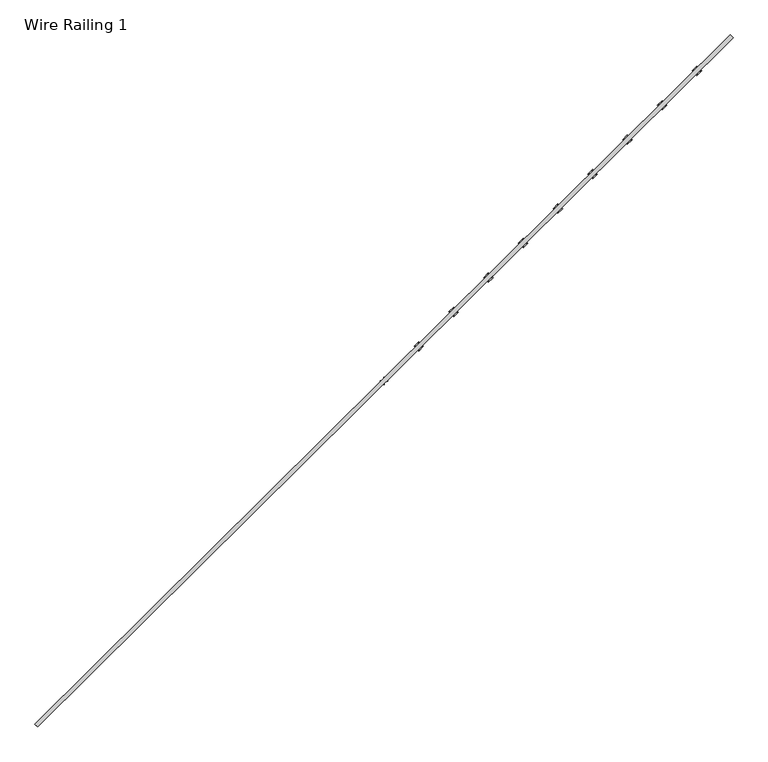
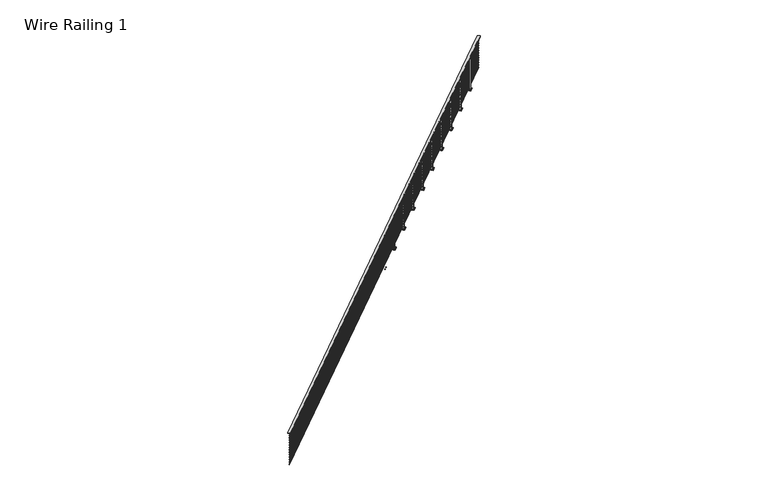
"""IFC4 building model written with IfcOpenShell, lengths in millimetres: railing geometry, Wire Railing 1."""

from ifc_helpers import new_model, si_unit, point, frame, frame_2d, origin, place, context, project, spatial, polyline, circle_curve, trimmed, segment, composite_curve, outline, extrude, source, transform, mapped, element, save


def wire_railing_1_bdb17c3e(model_context):
    return source(origin(), model_context, "Body", "SweptSolid", [
        extrude(outline(polyline([(32583.8298074, 24310.825617), (32530.1909697, 24364.9487644), (45743.1001377, 37459.6249857), (45796.7389755, 37405.5018383), (32583.8298074, 24310.825617)])), frame((0.0, 0.0, 265004.55), z_axis=(0.0, 0.0, 1.0), x_axis=(1.0, 0.0, 0.0)), (0.0, 0.0, 1.0), 19.05),
        extrude(outline(composite_curve([segment(trimmed(circle_curve(frame_2d((0.0, 2.38125)), 2.38125), [point((-2.38125, 2.38125))], [point((2.38125, 2.38125))], False, "CARTESIAN"), True, "CONTINUOUS"), segment(trimmed(circle_curve(frame_2d((0.0, 2.38125)), 2.38125), [point((2.38125, 2.38125))], [point((-2.38125, 2.38125))], False, "CARTESIAN"), True, "CONTINUOUS")], self_intersect=False)), frame((32557.0103886, 24337.8871907, 264947.4), z_axis=(0.7102775248505508, 0.7039217553763878, 0.0), x_axis=(0.7039217553763878, -0.7102775248505508, 0.0)), (0.0, 0.0, 1.0), 18602.4598918),
        extrude(outline(composite_curve([segment(trimmed(circle_curve(frame_2d((0.0, 2.38125)), 2.38125), [point((-2.38125, 2.38125))], [point((2.38125, 2.38125))], False, "CARTESIAN"), True, "CONTINUOUS"), segment(trimmed(circle_curve(frame_2d((0.0, 2.38125)), 2.38125), [point((2.38125, 2.38125))], [point((-2.38125, 2.38125))], False, "CARTESIAN"), True, "CONTINUOUS")], self_intersect=False)), frame((32557.0103886, 24337.8871907, 264871.2), z_axis=(0.7102775248505508, 0.7039217553763878, 0.0), x_axis=(0.7039217553763878, -0.7102775248505508, 0.0)), (0.0, 0.0, 1.0), 18602.4598918),
        extrude(outline(composite_curve([segment(trimmed(circle_curve(frame_2d((0.0, 2.38125)), 2.38125), [point((-2.38125, 2.38125))], [point((2.38125, 2.38125))], False, "CARTESIAN"), True, "CONTINUOUS"), segment(trimmed(circle_curve(frame_2d((0.0, 2.38125)), 2.38125), [point((2.38125, 2.38125))], [point((-2.38125, 2.38125))], False, "CARTESIAN"), True, "CONTINUOUS")], self_intersect=False)), frame((32557.0103886, 24337.8871907, 264795.0), z_axis=(0.7102775248505508, 0.7039217553763878, 0.0), x_axis=(0.7039217553763878, -0.7102775248505508, 0.0)), (0.0, 0.0, 1.0), 18602.4598918),
        extrude(outline(composite_curve([segment(trimmed(circle_curve(frame_2d((0.0, 2.38125)), 2.38125), [point((-2.38125, 2.38125))], [point((2.38125, 2.38125))], False, "CARTESIAN"), True, "CONTINUOUS"), segment(trimmed(circle_curve(frame_2d((0.0, 2.38125)), 2.38125), [point((2.38125, 2.38125))], [point((-2.38125, 2.38125))], False, "CARTESIAN"), True, "CONTINUOUS")], self_intersect=False)), frame((32557.0103886, 24337.8871907, 264718.8), z_axis=(0.7102775248505508, 0.7039217553763878, 0.0), x_axis=(0.7039217553763878, -0.7102775248505508, 0.0)), (0.0, 0.0, 1.0), 18602.4598918),
        extrude(outline(composite_curve([segment(trimmed(circle_curve(frame_2d((0.0, 2.38125)), 2.38125), [point((-2.38125, 2.38125))], [point((2.38125, 2.38125))], False, "CARTESIAN"), True, "CONTINUOUS"), segment(trimmed(circle_curve(frame_2d((0.0, 2.38125)), 2.38125), [point((2.38125, 2.38125))], [point((-2.38125, 2.38125))], False, "CARTESIAN"), True, "CONTINUOUS")], self_intersect=False)), frame((32557.0103886, 24337.8871907, 264642.6), z_axis=(0.7102775248505508, 0.7039217553763878, 0.0), x_axis=(0.7039217553763878, -0.7102775248505508, 0.0)), (0.0, 0.0, 1.0), 18602.4598918),
        extrude(outline(composite_curve([segment(trimmed(circle_curve(frame_2d((0.0, 2.38125)), 2.38125), [point((-2.38125, 2.38125))], [point((2.38125, 2.38125))], False, "CARTESIAN"), True, "CONTINUOUS"), segment(trimmed(circle_curve(frame_2d((0.0, 2.38125)), 2.38125), [point((2.38125, 2.38125))], [point((-2.38125, 2.38125))], False, "CARTESIAN"), True, "CONTINUOUS")], self_intersect=False)), frame((32557.0103886, 24337.8871907, 264566.4), z_axis=(0.7102775248505508, 0.7039217553763878, 0.0), x_axis=(0.7039217553763878, -0.7102775248505508, 0.0)), (0.0, 0.0, 1.0), 18602.4598918),
        extrude(outline(composite_curve([segment(trimmed(circle_curve(frame_2d((0.0, 2.38125)), 2.38125), [point((-2.38125, 2.38125))], [point((2.38125, 2.38125))], False, "CARTESIAN"), True, "CONTINUOUS"), segment(trimmed(circle_curve(frame_2d((0.0, 2.38125)), 2.38125), [point((2.38125, 2.38125))], [point((-2.38125, 2.38125))], False, "CARTESIAN"), True, "CONTINUOUS")], self_intersect=False)), frame((32557.0103886, 24337.8871907, 264490.2), z_axis=(0.7102775248505508, 0.7039217553763878, 0.0), x_axis=(0.7039217553763878, -0.7102775248505508, 0.0)), (0.0, 0.0, 1.0), 18602.4598918),
        extrude(outline(composite_curve([segment(trimmed(circle_curve(frame_2d((0.0, 2.38125)), 2.38125), [point((-2.38125, 2.38125))], [point((2.38125, 2.38125))], False, "CARTESIAN"), True, "CONTINUOUS"), segment(trimmed(circle_curve(frame_2d((0.0, 2.38125)), 2.38125), [point((2.38125, 2.38125))], [point((-2.38125, 2.38125))], False, "CARTESIAN"), True, "CONTINUOUS")], self_intersect=False)), frame((32557.0103886, 24337.8871907, 264414.0), z_axis=(0.7102775248505508, 0.7039217553763878, 0.0), x_axis=(0.7039217553763878, -0.7102775248505508, 0.0)), (0.0, 0.0, 1.0), 18602.4598918),
        extrude(outline(composite_curve([segment(trimmed(circle_curve(frame_2d((0.0, 2.38125)), 2.38125), [point((-2.38125, 2.38125))], [point((2.38125, 2.38125))], False, "CARTESIAN"), True, "CONTINUOUS"), segment(trimmed(circle_curve(frame_2d((0.0, 2.38125)), 2.38125), [point((2.38125, 2.38125))], [point((-2.38125, 2.38125))], False, "CARTESIAN"), True, "CONTINUOUS")], self_intersect=False)), frame((32557.0103886, 24337.8871907, 264337.8), z_axis=(0.7102775248505508, 0.7039217553763878, 0.0), x_axis=(0.7039217553763878, -0.7102775248505508, 0.0)), (0.0, 0.0, 1.0), 18602.4598918),
        extrude(outline(composite_curve([segment(trimmed(circle_curve(frame_2d((0.0, 2.38125)), 2.38125), [point((-2.38125, 2.38125))], [point((2.38125, 2.38125))], False, "CARTESIAN"), True, "CONTINUOUS"), segment(trimmed(circle_curve(frame_2d((0.0, 2.38125)), 2.38125), [point((2.38125, 2.38125))], [point((-2.38125, 2.38125))], False, "CARTESIAN"), True, "CONTINUOUS")], self_intersect=False)), frame((32557.0103886, 24337.8871907, 264261.6), z_axis=(0.7102775248505508, 0.7039217553763878, 0.0), x_axis=(0.7039217553763878, -0.7102775248505508, 0.0)), (0.0, 0.0, 1.0), 18602.4598918),
        extrude(outline(composite_curve([segment(trimmed(circle_curve(frame_2d((0.0, 2.38125)), 2.38125), [point((-2.38125, 2.38125))], [point((2.38125, 2.38125))], False, "CARTESIAN"), True, "CONTINUOUS"), segment(trimmed(circle_curve(frame_2d((0.0, 2.38125)), 2.38125), [point((2.38125, 2.38125))], [point((-2.38125, 2.38125))], False, "CARTESIAN"), True, "CONTINUOUS")], self_intersect=False)), frame((32557.0103886, 24337.8871907, 264185.4), z_axis=(0.7102775248505508, 0.7039217553763878, 0.0), x_axis=(0.7039217553763878, -0.7102775248505508, 0.0)), (0.0, 0.0, 1.0), 18602.4598918),
        extrude(outline(composite_curve([segment(trimmed(circle_curve(frame_2d((0.0, 2.38125)), 2.38125), [point((-2.38125, 2.38125))], [point((2.38125, 2.38125))], False, "CARTESIAN"), True, "CONTINUOUS"), segment(trimmed(circle_curve(frame_2d((0.0, 2.38125)), 2.38125), [point((2.38125, 2.38125))], [point((-2.38125, 2.38125))], False, "CARTESIAN"), True, "CONTINUOUS")], self_intersect=False)), frame((32557.0103886, 24337.8871907, 264109.2), z_axis=(0.7102775248505508, 0.7039217553763878, 0.0), x_axis=(0.7039217553763878, -0.7102775248505508, 0.0)), (0.0, 0.0, 1.0), 18602.4598918),
        extrude(outline(composite_curve([segment(trimmed(circle_curve(frame_2d((0.0, 2.38125)), 2.38125), [point((-2.38125, 2.38125))], [point((2.38125, 2.38125))], False, "CARTESIAN"), True, "CONTINUOUS"), segment(trimmed(circle_curve(frame_2d((0.0, 2.38125)), 2.38125), [point((2.38125, 2.38125))], [point((-2.38125, 2.38125))], False, "CARTESIAN"), True, "CONTINUOUS")], self_intersect=False)), frame((32557.0103886, 24337.8871907, 264033.0), z_axis=(0.7102775248505508, 0.7039217553763878, 0.0), x_axis=(0.7039217553763878, -0.7102775248505508, 0.0)), (0.0, 0.0, 1.0), 18602.4598918),
        extrude(outline(composite_curve([segment(trimmed(circle_curve(frame_2d((45108.9915842, 36714.968443)), 6.35), [point((45113.4614874, 36710.4581807))], [point((45104.5216811, 36719.4787052))], False, "CARTESIAN"), True, "CONTINUOUS"), segment(trimmed(circle_curve(frame_2d((45108.9915842, 36714.968443)), 6.35), [point((45104.5216811, 36719.4787052))], [point((45113.4614874, 36710.4581807))], False, "CARTESIAN"), True, "CONTINUOUS")], self_intersect=False)), frame((0.0, 0.0, 263956.8), z_axis=(0.0, 0.0, 1.0), x_axis=(1.0, 0.0, 0.0)), (0.0, 0.0, 1.0), 12.7),
        extrude(outline(composite_curve([segment(trimmed(circle_curve(frame_2d((45046.4129402, 36778.1121149)), 6.35), [point((45050.8828433, 36773.6018526))], [point((45041.943037, 36782.6223772))], False, "CARTESIAN"), True, "CONTINUOUS"), segment(trimmed(circle_curve(frame_2d((45046.4129402, 36778.1121149)), 6.35), [point((45041.943037, 36782.6223772))], [point((45050.8828433, 36773.6018526))], False, "CARTESIAN"), True, "CONTINUOUS")], self_intersect=False)), frame((0.0, 0.0, 263956.8), z_axis=(0.0, 0.0, 1.0), x_axis=(1.0, 0.0, 0.0)), (0.0, 0.0, 1.0), 12.7),
        extrude(outline(composite_curve([segment(trimmed(circle_curve(frame_2d((45172.1352562, 36777.547087)), 6.35), [point((45176.6051594, 36773.0368247))], [point((45167.6653531, 36782.0573493))], False, "CARTESIAN"), True, "CONTINUOUS"), segment(trimmed(circle_curve(frame_2d((45172.1352562, 36777.547087)), 6.35), [point((45167.6653531, 36782.0573493))], [point((45176.6051594, 36773.0368247))], False, "CARTESIAN"), True, "CONTINUOUS")], self_intersect=False)), frame((0.0, 0.0, 263956.8), z_axis=(0.0, 0.0, 1.0), x_axis=(1.0, 0.0, 0.0)), (0.0, 0.0, 1.0), 12.7),
        extrude(outline(composite_curve([segment(trimmed(circle_curve(frame_2d((45109.5566122, 36840.690759)), 6.35), [point((45114.0265153, 36836.1804967))], [point((45105.086709, 36845.2010212))], False, "CARTESIAN"), True, "CONTINUOUS"), segment(trimmed(circle_curve(frame_2d((45109.5566122, 36840.690759)), 6.35), [point((45105.086709, 36845.2010212))], [point((45114.0265153, 36836.1804967))], False, "CARTESIAN"), True, "CONTINUOUS")], self_intersect=False)), frame((0.0, 0.0, 263956.8), z_axis=(0.0, 0.0, 1.0), x_axis=(1.0, 0.0, 0.0)), (0.0, 0.0, 1.0), 12.7),
        extrude(outline(polyline([(45019.4724439, 36778.2331923), (45109.6776896, 36867.6312553), (45199.0757525, 36777.4260096), (45108.8705068, 36688.0279467), (45019.4724439, 36778.2331923)])), frame((0.0, 0.0, 263956.8), z_axis=(0.0, 0.0, 1.0), x_axis=(1.0, 0.0, 0.0)), (0.0, 0.0, 1.0), 6.35),
        extrude(outline(polyline([(45066.6183124, 36778.0213069), (45109.4658041, 36820.4853867), (45151.929884, 36777.6378951), (45109.0823923, 36735.1738152), (45066.6183124, 36778.0213069)]), holes=[polyline([(45075.5984778, 36777.9809477), (45109.1227514, 36744.1539806), (45142.9497186, 36777.6782542), (45109.425445, 36811.5052213), (45075.5984778, 36777.9809477)])]), frame((0.0, 0.0, 263956.8), z_axis=(0.0, 0.0, 1.0), x_axis=(1.0, 0.0, 0.0)), (0.0, 0.0, 1.0), 1047.75),
        extrude(outline(composite_curve([segment(trimmed(circle_curve(frame_2d((44448.3461258, 36060.2346319)), 6.35), [point((44452.816029, 36055.7243696))], [point((44443.8762227, 36064.7448942))], False, "CARTESIAN"), True, "CONTINUOUS"), segment(trimmed(circle_curve(frame_2d((44448.3461258, 36060.2346319)), 6.35), [point((44443.8762227, 36064.7448942))], [point((44452.816029, 36055.7243696))], False, "CARTESIAN"), True, "CONTINUOUS")], self_intersect=False)), frame((0.0, 0.0, 263956.8), z_axis=(0.0, 0.0, 1.0), x_axis=(1.0, 0.0, 0.0)), (0.0, 0.0, 1.0), 12.7),
        extrude(outline(composite_curve([segment(trimmed(circle_curve(frame_2d((44385.7674818, 36123.3783038)), 6.35), [point((44390.2373849, 36118.8680416))], [point((44381.2975786, 36127.8885661))], False, "CARTESIAN"), True, "CONTINUOUS"), segment(trimmed(circle_curve(frame_2d((44385.7674818, 36123.3783038)), 6.35), [point((44381.2975786, 36127.8885661))], [point((44390.2373849, 36118.8680416))], False, "CARTESIAN"), True, "CONTINUOUS")], self_intersect=False)), frame((0.0, 0.0, 263956.8), z_axis=(0.0, 0.0, 1.0), x_axis=(1.0, 0.0, 0.0)), (0.0, 0.0, 1.0), 12.7),
        extrude(outline(composite_curve([segment(trimmed(circle_curve(frame_2d((44511.4897978, 36122.8132759)), 6.35), [point((44515.959701, 36118.3030137))], [point((44507.0198947, 36127.3235382))], False, "CARTESIAN"), True, "CONTINUOUS"), segment(trimmed(circle_curve(frame_2d((44511.4897978, 36122.8132759)), 6.35), [point((44507.0198947, 36127.3235382))], [point((44515.959701, 36118.3030137))], False, "CARTESIAN"), True, "CONTINUOUS")], self_intersect=False)), frame((0.0, 0.0, 263956.8), z_axis=(0.0, 0.0, 1.0), x_axis=(1.0, 0.0, 0.0)), (0.0, 0.0, 1.0), 12.7),
        extrude(outline(composite_curve([segment(trimmed(circle_curve(frame_2d((44448.9111538, 36185.9569479)), 6.35), [point((44453.3810569, 36181.4466856))], [point((44444.4412506, 36190.4672102))], False, "CARTESIAN"), True, "CONTINUOUS"), segment(trimmed(circle_curve(frame_2d((44448.9111538, 36185.9569479)), 6.35), [point((44444.4412506, 36190.4672102))], [point((44453.3810569, 36181.4466856))], False, "CARTESIAN"), True, "CONTINUOUS")], self_intersect=False)), frame((0.0, 0.0, 263956.8), z_axis=(0.0, 0.0, 1.0), x_axis=(1.0, 0.0, 0.0)), (0.0, 0.0, 1.0), 12.7),
        extrude(outline(polyline([(44358.8269855, 36123.4993813), (44449.0322312, 36212.8974442), (44538.4302941, 36122.6921985), (44448.2250484, 36033.2941356), (44358.8269855, 36123.4993813)])), frame((0.0, 0.0, 263956.8), z_axis=(0.0, 0.0, 1.0), x_axis=(1.0, 0.0, 0.0)), (0.0, 0.0, 1.0), 6.35),
        extrude(outline(polyline([(44405.972854, 36123.2874958), (44448.8203457, 36165.7515757), (44491.2844256, 36122.904084), (44448.4369339, 36080.4400041), (44405.972854, 36123.2874958)]), holes=[polyline([(44414.9530194, 36123.2471367), (44448.477293, 36089.4201695), (44482.3042602, 36122.9444431), (44448.7799866, 36156.7714103), (44414.9530194, 36123.2471367)])]), frame((0.0, 0.0, 263956.8), z_axis=(0.0, 0.0, 1.0), x_axis=(1.0, 0.0, 0.0)), (0.0, 0.0, 1.0), 1047.75),
        extrude(outline(composite_curve([segment(trimmed(circle_curve(frame_2d((43787.7006674, 35405.5008208)), 6.35), [point((43792.1705706, 35400.9905585))], [point((43783.2307643, 35410.0110831))], False, "CARTESIAN"), True, "CONTINUOUS"), segment(trimmed(circle_curve(frame_2d((43787.7006674, 35405.5008208)), 6.35), [point((43783.2307643, 35410.0110831))], [point((43792.1705706, 35400.9905585))], False, "CARTESIAN"), True, "CONTINUOUS")], self_intersect=False)), frame((0.0, 0.0, 263956.8), z_axis=(0.0, 0.0, 1.0), x_axis=(1.0, 0.0, 0.0)), (0.0, 0.0, 1.0), 12.7),
        extrude(outline(composite_curve([segment(trimmed(circle_curve(frame_2d((43725.1220234, 35468.6444928)), 6.35), [point((43729.5919265, 35464.1342305))], [point((43720.6521202, 35473.1547551))], False, "CARTESIAN"), True, "CONTINUOUS"), segment(trimmed(circle_curve(frame_2d((43725.1220234, 35468.6444928)), 6.35), [point((43720.6521202, 35473.1547551))], [point((43729.5919265, 35464.1342305))], False, "CARTESIAN"), True, "CONTINUOUS")], self_intersect=False)), frame((0.0, 0.0, 263956.8), z_axis=(0.0, 0.0, 1.0), x_axis=(1.0, 0.0, 0.0)), (0.0, 0.0, 1.0), 12.7),
        extrude(outline(composite_curve([segment(trimmed(circle_curve(frame_2d((43850.8443394, 35468.0794649)), 6.35), [point((43855.3142425, 35463.5692026))], [point((43846.3744363, 35472.5897272))], False, "CARTESIAN"), True, "CONTINUOUS"), segment(trimmed(circle_curve(frame_2d((43850.8443394, 35468.0794649)), 6.35), [point((43846.3744363, 35472.5897272))], [point((43855.3142425, 35463.5692026))], False, "CARTESIAN"), True, "CONTINUOUS")], self_intersect=False)), frame((0.0, 0.0, 263956.8), z_axis=(0.0, 0.0, 1.0), x_axis=(1.0, 0.0, 0.0)), (0.0, 0.0, 1.0), 12.7),
        extrude(outline(composite_curve([segment(trimmed(circle_curve(frame_2d((43788.2656953, 35531.2231368)), 6.35), [point((43792.7355985, 35526.7128745))], [point((43783.7957922, 35535.7333991))], False, "CARTESIAN"), True, "CONTINUOUS"), segment(trimmed(circle_curve(frame_2d((43788.2656953, 35531.2231368)), 6.35), [point((43783.7957922, 35535.7333991))], [point((43792.7355985, 35526.7128745))], False, "CARTESIAN"), True, "CONTINUOUS")], self_intersect=False)), frame((0.0, 0.0, 263956.8), z_axis=(0.0, 0.0, 1.0), x_axis=(1.0, 0.0, 0.0)), (0.0, 0.0, 1.0), 12.7),
        extrude(outline(polyline([(43698.1815271, 35468.7655702), (43788.3867728, 35558.1636331), (43877.7848357, 35467.9583875), (43787.57959, 35378.5603245), (43698.1815271, 35468.7655702)])), frame((0.0, 0.0, 263956.8), z_axis=(0.0, 0.0, 1.0), x_axis=(1.0, 0.0, 0.0)), (0.0, 0.0, 1.0), 6.35),
        extrude(outline(polyline([(43745.3273956, 35468.5536847), (43788.1748873, 35511.0177646), (43830.6389672, 35468.1702729), (43787.7914755, 35425.706193), (43745.3273956, 35468.5536847)]), holes=[polyline([(43754.307561, 35468.5133256), (43787.8318346, 35434.6863585), (43821.6588018, 35468.2106321), (43788.1345282, 35502.0375992), (43754.307561, 35468.5133256)])]), frame((0.0, 0.0, 263956.8), z_axis=(0.0, 0.0, 1.0), x_axis=(1.0, 0.0, 0.0)), (0.0, 0.0, 1.0), 1047.75),
        extrude(outline(composite_curve([segment(trimmed(circle_curve(frame_2d((43127.055209, 34750.7670098)), 6.35), [point((43131.5251122, 34746.2567475))], [point((43122.5853059, 34755.277272))], False, "CARTESIAN"), True, "CONTINUOUS"), segment(trimmed(circle_curve(frame_2d((43127.055209, 34750.7670098)), 6.35), [point((43122.5853059, 34755.277272))], [point((43131.5251122, 34746.2567475))], False, "CARTESIAN"), True, "CONTINUOUS")], self_intersect=False)), frame((0.0, 0.0, 263956.8), z_axis=(0.0, 0.0, 1.0), x_axis=(1.0, 0.0, 0.0)), (0.0, 0.0, 1.0), 12.7),
        extrude(outline(composite_curve([segment(trimmed(circle_curve(frame_2d((43064.476565, 34813.9106817)), 6.35), [point((43068.9464681, 34809.4004194))], [point((43060.0066618, 34818.420944))], False, "CARTESIAN"), True, "CONTINUOUS"), segment(trimmed(circle_curve(frame_2d((43064.476565, 34813.9106817)), 6.35), [point((43060.0066618, 34818.420944))], [point((43068.9464681, 34809.4004194))], False, "CARTESIAN"), True, "CONTINUOUS")], self_intersect=False)), frame((0.0, 0.0, 263956.8), z_axis=(0.0, 0.0, 1.0), x_axis=(1.0, 0.0, 0.0)), (0.0, 0.0, 1.0), 12.7),
        extrude(outline(composite_curve([segment(trimmed(circle_curve(frame_2d((43190.198881, 34813.3456538)), 6.35), [point((43194.6687841, 34808.8353915))], [point((43185.7289779, 34817.8559161))], False, "CARTESIAN"), True, "CONTINUOUS"), segment(trimmed(circle_curve(frame_2d((43190.198881, 34813.3456538)), 6.35), [point((43185.7289779, 34817.8559161))], [point((43194.6687841, 34808.8353915))], False, "CARTESIAN"), True, "CONTINUOUS")], self_intersect=False)), frame((0.0, 0.0, 263956.8), z_axis=(0.0, 0.0, 1.0), x_axis=(1.0, 0.0, 0.0)), (0.0, 0.0, 1.0), 12.7),
        extrude(outline(composite_curve([segment(trimmed(circle_curve(frame_2d((43127.6202369, 34876.4893258)), 6.35), [point((43132.0901401, 34871.9790635))], [point((43123.1503338, 34880.999588))], False, "CARTESIAN"), True, "CONTINUOUS"), segment(trimmed(circle_curve(frame_2d((43127.6202369, 34876.4893258)), 6.35), [point((43123.1503338, 34880.999588))], [point((43132.0901401, 34871.9790635))], False, "CARTESIAN"), True, "CONTINUOUS")], self_intersect=False)), frame((0.0, 0.0, 263956.8), z_axis=(0.0, 0.0, 1.0), x_axis=(1.0, 0.0, 0.0)), (0.0, 0.0, 1.0), 12.7),
        extrude(outline(polyline([(43037.5360687, 34814.0317591), (43127.7413144, 34903.4298221), (43217.1393773, 34813.2245764), (43126.9341316, 34723.8265135), (43037.5360687, 34814.0317591)])), frame((0.0, 0.0, 263956.8), z_axis=(0.0, 0.0, 1.0), x_axis=(1.0, 0.0, 0.0)), (0.0, 0.0, 1.0), 6.35),
        extrude(outline(polyline([(43084.6819372, 34813.8198737), (43127.5294289, 34856.2839535), (43169.9935088, 34813.4364619), (43127.1460171, 34770.972382), (43084.6819372, 34813.8198737)]), holes=[polyline([(43093.6621026, 34813.7795145), (43127.1863762, 34779.9525474), (43161.0133434, 34813.476821), (43127.4890698, 34847.3037881), (43093.6621026, 34813.7795145)])]), frame((0.0, 0.0, 263956.8), z_axis=(0.0, 0.0, 1.0), x_axis=(1.0, 0.0, 0.0)), (0.0, 0.0, 1.0), 1047.75),
        extrude(outline(composite_curve([segment(trimmed(circle_curve(frame_2d((42466.4097506, 34096.0331987)), 6.35), [point((42470.8796538, 34091.5229364))], [point((42461.9398475, 34100.543461))], False, "CARTESIAN"), True, "CONTINUOUS"), segment(trimmed(circle_curve(frame_2d((42466.4097506, 34096.0331987)), 6.35), [point((42461.9398475, 34100.543461))], [point((42470.8796538, 34091.5229364))], False, "CARTESIAN"), True, "CONTINUOUS")], self_intersect=False)), frame((0.0, 0.0, 263956.8), z_axis=(0.0, 0.0, 1.0), x_axis=(1.0, 0.0, 0.0)), (0.0, 0.0, 1.0), 12.7),
        extrude(outline(composite_curve([segment(trimmed(circle_curve(frame_2d((42403.8311066, 34159.1768706)), 6.35), [point((42408.3010097, 34154.6666084))], [point((42399.3612034, 34163.6871329))], False, "CARTESIAN"), True, "CONTINUOUS"), segment(trimmed(circle_curve(frame_2d((42403.8311066, 34159.1768706)), 6.35), [point((42399.3612034, 34163.6871329))], [point((42408.3010097, 34154.6666084))], False, "CARTESIAN"), True, "CONTINUOUS")], self_intersect=False)), frame((0.0, 0.0, 263956.8), z_axis=(0.0, 0.0, 1.0), x_axis=(1.0, 0.0, 0.0)), (0.0, 0.0, 1.0), 12.7),
        extrude(outline(composite_curve([segment(trimmed(circle_curve(frame_2d((42529.5534226, 34158.6118427)), 6.35), [point((42534.0233257, 34154.1015805))], [point((42525.0835195, 34163.122105))], False, "CARTESIAN"), True, "CONTINUOUS"), segment(trimmed(circle_curve(frame_2d((42529.5534226, 34158.6118427)), 6.35), [point((42525.0835195, 34163.122105))], [point((42534.0233257, 34154.1015805))], False, "CARTESIAN"), True, "CONTINUOUS")], self_intersect=False)), frame((0.0, 0.0, 263956.8), z_axis=(0.0, 0.0, 1.0), x_axis=(1.0, 0.0, 0.0)), (0.0, 0.0, 1.0), 12.7),
        extrude(outline(composite_curve([segment(trimmed(circle_curve(frame_2d((42466.9747785, 34221.7555147)), 6.35), [point((42471.4446817, 34217.2452524))], [point((42462.5048754, 34226.265777))], False, "CARTESIAN"), True, "CONTINUOUS"), segment(trimmed(circle_curve(frame_2d((42466.9747785, 34221.7555147)), 6.35), [point((42462.5048754, 34226.265777))], [point((42471.4446817, 34217.2452524))], False, "CARTESIAN"), True, "CONTINUOUS")], self_intersect=False)), frame((0.0, 0.0, 263956.8), z_axis=(0.0, 0.0, 1.0), x_axis=(1.0, 0.0, 0.0)), (0.0, 0.0, 1.0), 12.7),
        extrude(outline(polyline([(42376.8906103, 34159.2979481), (42467.095856, 34248.696011), (42556.4939189, 34158.4907653), (42466.2886732, 34069.0927024), (42376.8906103, 34159.2979481)])), frame((0.0, 0.0, 263956.8), z_axis=(0.0, 0.0, 1.0), x_axis=(1.0, 0.0, 0.0)), (0.0, 0.0, 1.0), 6.35),
        extrude(outline(polyline([(42424.0364788, 34159.0860626), (42466.8839705, 34201.5501425), (42509.3480504, 34158.7026508), (42466.5005587, 34116.2385709), (42424.0364788, 34159.0860626)]), holes=[polyline([(42433.0166442, 34159.0457035), (42466.5409178, 34125.2187363), (42500.367885, 34158.7430099), (42466.8436114, 34192.5699771), (42433.0166442, 34159.0457035)])]), frame((0.0, 0.0, 263956.8), z_axis=(0.0, 0.0, 1.0), x_axis=(1.0, 0.0, 0.0)), (0.0, 0.0, 1.0), 1047.75),
        extrude(outline(composite_curve([segment(trimmed(circle_curve(frame_2d((41805.7642922, 33441.2993876)), 6.35), [point((41810.2341954, 33436.7891253))], [point((41801.2943891, 33445.8096499))], False, "CARTESIAN"), True, "CONTINUOUS"), segment(trimmed(circle_curve(frame_2d((41805.7642922, 33441.2993876)), 6.35), [point((41801.2943891, 33445.8096499))], [point((41810.2341954, 33436.7891253))], False, "CARTESIAN"), True, "CONTINUOUS")], self_intersect=False)), frame((0.0, 0.0, 263956.8), z_axis=(0.0, 0.0, 1.0), x_axis=(1.0, 0.0, 0.0)), (0.0, 0.0, 1.0), 12.7),
        extrude(outline(composite_curve([segment(trimmed(circle_curve(frame_2d((41743.1856482, 33504.4430596)), 6.35), [point((41747.6555513, 33499.9327973))], [point((41738.715745, 33508.9533219))], False, "CARTESIAN"), True, "CONTINUOUS"), segment(trimmed(circle_curve(frame_2d((41743.1856482, 33504.4430596)), 6.35), [point((41738.715745, 33508.9533219))], [point((41747.6555513, 33499.9327973))], False, "CARTESIAN"), True, "CONTINUOUS")], self_intersect=False)), frame((0.0, 0.0, 263956.8), z_axis=(0.0, 0.0, 1.0), x_axis=(1.0, 0.0, 0.0)), (0.0, 0.0, 1.0), 12.7),
        extrude(outline(composite_curve([segment(trimmed(circle_curve(frame_2d((41868.9079642, 33503.8780317)), 6.35), [point((41873.3778673, 33499.3677694))], [point((41864.438061, 33508.388294))], False, "CARTESIAN"), True, "CONTINUOUS"), segment(trimmed(circle_curve(frame_2d((41868.9079642, 33503.8780317)), 6.35), [point((41864.438061, 33508.388294))], [point((41873.3778673, 33499.3677694))], False, "CARTESIAN"), True, "CONTINUOUS")], self_intersect=False)), frame((0.0, 0.0, 263956.8), z_axis=(0.0, 0.0, 1.0), x_axis=(1.0, 0.0, 0.0)), (0.0, 0.0, 1.0), 12.7),
        extrude(outline(composite_curve([segment(trimmed(circle_curve(frame_2d((41806.3293201, 33567.0217036)), 6.35), [point((41810.7992233, 33562.5114413))], [point((41801.859417, 33571.5319659))], False, "CARTESIAN"), True, "CONTINUOUS"), segment(trimmed(circle_curve(frame_2d((41806.3293201, 33567.0217036)), 6.35), [point((41801.859417, 33571.5319659))], [point((41810.7992233, 33562.5114413))], False, "CARTESIAN"), True, "CONTINUOUS")], self_intersect=False)), frame((0.0, 0.0, 263956.8), z_axis=(0.0, 0.0, 1.0), x_axis=(1.0, 0.0, 0.0)), (0.0, 0.0, 1.0), 12.7),
        extrude(outline(polyline([(41716.2451519, 33504.564137), (41806.4503975, 33593.9621999), (41895.8484605, 33503.7569543), (41805.6432148, 33414.3588913), (41716.2451519, 33504.564137)])), frame((0.0, 0.0, 263956.8), z_axis=(0.0, 0.0, 1.0), x_axis=(1.0, 0.0, 0.0)), (0.0, 0.0, 1.0), 6.35),
        extrude(outline(polyline([(41763.3910204, 33504.3522515), (41806.2385121, 33546.8163314), (41848.702592, 33503.9688397), (41805.8551003, 33461.5047598), (41763.3910204, 33504.3522515)]), holes=[polyline([(41772.3711858, 33504.3118924), (41805.8954594, 33470.4849253), (41839.7224265, 33504.0091989), (41806.1981529, 33537.836166), (41772.3711858, 33504.3118924)])]), frame((0.0, 0.0, 263956.8), z_axis=(0.0, 0.0, 1.0), x_axis=(1.0, 0.0, 0.0)), (0.0, 0.0, 1.0), 1047.75),
        extrude(outline(composite_curve([segment(trimmed(circle_curve(frame_2d((41145.1188338, 32786.5655766)), 6.35), [point((41149.588737, 32782.0553143))], [point((41140.6489307, 32791.0758388))], False, "CARTESIAN"), True, "CONTINUOUS"), segment(trimmed(circle_curve(frame_2d((41145.1188338, 32786.5655766)), 6.35), [point((41140.6489307, 32791.0758388))], [point((41149.588737, 32782.0553143))], False, "CARTESIAN"), True, "CONTINUOUS")], self_intersect=False)), frame((0.0, 0.0, 263956.8), z_axis=(0.0, 0.0, 1.0), x_axis=(1.0, 0.0, 0.0)), (0.0, 0.0, 1.0), 12.7),
        extrude(outline(composite_curve([segment(trimmed(circle_curve(frame_2d((41082.5401898, 32849.7092485)), 6.35), [point((41087.0100929, 32845.1989862))], [point((41078.0702866, 32854.2195108))], False, "CARTESIAN"), True, "CONTINUOUS"), segment(trimmed(circle_curve(frame_2d((41082.5401898, 32849.7092485)), 6.35), [point((41078.0702866, 32854.2195108))], [point((41087.0100929, 32845.1989862))], False, "CARTESIAN"), True, "CONTINUOUS")], self_intersect=False)), frame((0.0, 0.0, 263956.8), z_axis=(0.0, 0.0, 1.0), x_axis=(1.0, 0.0, 0.0)), (0.0, 0.0, 1.0), 12.7),
        extrude(outline(composite_curve([segment(trimmed(circle_curve(frame_2d((41208.2625058, 32849.1442206)), 6.35), [point((41212.7324089, 32844.6339583))], [point((41203.7926026, 32853.6544829))], False, "CARTESIAN"), True, "CONTINUOUS"), segment(trimmed(circle_curve(frame_2d((41208.2625058, 32849.1442206)), 6.35), [point((41203.7926026, 32853.6544829))], [point((41212.7324089, 32844.6339583))], False, "CARTESIAN"), True, "CONTINUOUS")], self_intersect=False)), frame((0.0, 0.0, 263956.8), z_axis=(0.0, 0.0, 1.0), x_axis=(1.0, 0.0, 0.0)), (0.0, 0.0, 1.0), 12.7),
        extrude(outline(composite_curve([segment(trimmed(circle_curve(frame_2d((41145.6838617, 32912.2878926)), 6.35), [point((41150.1537649, 32907.7776303))], [point((41141.2139586, 32916.7981548))], False, "CARTESIAN"), True, "CONTINUOUS"), segment(trimmed(circle_curve(frame_2d((41145.6838617, 32912.2878926)), 6.35), [point((41141.2139586, 32916.7981548))], [point((41150.1537649, 32907.7776303))], False, "CARTESIAN"), True, "CONTINUOUS")], self_intersect=False)), frame((0.0, 0.0, 263956.8), z_axis=(0.0, 0.0, 1.0), x_axis=(1.0, 0.0, 0.0)), (0.0, 0.0, 1.0), 12.7),
        extrude(outline(polyline([(41055.5996935, 32849.8303259), (41145.8049391, 32939.2283889), (41235.2030021, 32849.0231432), (41144.9977564, 32759.6250803), (41055.5996935, 32849.8303259)])), frame((0.0, 0.0, 263956.8), z_axis=(0.0, 0.0, 1.0), x_axis=(1.0, 0.0, 0.0)), (0.0, 0.0, 1.0), 6.35),
        extrude(outline(polyline([(41102.745562, 32849.6184405), (41145.5930537, 32892.0825203), (41188.0571336, 32849.2350287), (41145.2096419, 32806.7709488), (41102.745562, 32849.6184405)]), holes=[polyline([(41111.7257274, 32849.5780813), (41145.250001, 32815.7511142), (41179.0769681, 32849.2753878), (41145.5526945, 32883.1023549), (41111.7257274, 32849.5780813)])]), frame((0.0, 0.0, 263956.8), z_axis=(0.0, 0.0, 1.0), x_axis=(1.0, 0.0, 0.0)), (0.0, 0.0, 1.0), 1047.75),
        extrude(outline(composite_curve([segment(trimmed(circle_curve(frame_2d((40484.4733754, 32131.8317655)), 6.35), [point((40488.9432786, 32127.3215032))], [point((40480.0034723, 32136.3420278))], False, "CARTESIAN"), True, "CONTINUOUS"), segment(trimmed(circle_curve(frame_2d((40484.4733754, 32131.8317655)), 6.35), [point((40480.0034723, 32136.3420278))], [point((40488.9432786, 32127.3215032))], False, "CARTESIAN"), True, "CONTINUOUS")], self_intersect=False)), frame((0.0, 0.0, 263956.8), z_axis=(0.0, 0.0, 1.0), x_axis=(1.0, 0.0, 0.0)), (0.0, 0.0, 1.0), 12.7),
        extrude(outline(composite_curve([segment(trimmed(circle_curve(frame_2d((40421.8947314, 32194.9754374)), 6.35), [point((40426.3646345, 32190.4651752))], [point((40417.4248282, 32199.4856997))], False, "CARTESIAN"), True, "CONTINUOUS"), segment(trimmed(circle_curve(frame_2d((40421.8947314, 32194.9754374)), 6.35), [point((40417.4248282, 32199.4856997))], [point((40426.3646345, 32190.4651752))], False, "CARTESIAN"), True, "CONTINUOUS")], self_intersect=False)), frame((0.0, 0.0, 263956.8), z_axis=(0.0, 0.0, 1.0), x_axis=(1.0, 0.0, 0.0)), (0.0, 0.0, 1.0), 12.7),
        extrude(outline(composite_curve([segment(trimmed(circle_curve(frame_2d((40547.6170474, 32194.4104095)), 6.35), [point((40552.0869505, 32189.9001473))], [point((40543.1471442, 32198.9206718))], False, "CARTESIAN"), True, "CONTINUOUS"), segment(trimmed(circle_curve(frame_2d((40547.6170474, 32194.4104095)), 6.35), [point((40543.1471442, 32198.9206718))], [point((40552.0869505, 32189.9001473))], False, "CARTESIAN"), True, "CONTINUOUS")], self_intersect=False)), frame((0.0, 0.0, 263956.8), z_axis=(0.0, 0.0, 1.0), x_axis=(1.0, 0.0, 0.0)), (0.0, 0.0, 1.0), 12.7),
        extrude(outline(composite_curve([segment(trimmed(circle_curve(frame_2d((40485.0384033, 32257.5540815)), 6.35), [point((40489.5083065, 32253.0438192))], [point((40480.5685002, 32262.0643438))], False, "CARTESIAN"), True, "CONTINUOUS"), segment(trimmed(circle_curve(frame_2d((40485.0384033, 32257.5540815)), 6.35), [point((40480.5685002, 32262.0643438))], [point((40489.5083065, 32253.0438192))], False, "CARTESIAN"), True, "CONTINUOUS")], self_intersect=False)), frame((0.0, 0.0, 263956.8), z_axis=(0.0, 0.0, 1.0), x_axis=(1.0, 0.0, 0.0)), (0.0, 0.0, 1.0), 12.7),
        extrude(outline(polyline([(40394.9542351, 32195.0965149), (40485.1594807, 32284.4945778), (40574.5575437, 32194.2893321), (40484.352298, 32104.8912692), (40394.9542351, 32195.0965149)])), frame((0.0, 0.0, 263956.8), z_axis=(0.0, 0.0, 1.0), x_axis=(1.0, 0.0, 0.0)), (0.0, 0.0, 1.0), 6.35),
        extrude(outline(polyline([(40442.1001036, 32194.8846294), (40484.9475953, 32237.3487093), (40527.4116752, 32194.5012176), (40484.5641835, 32152.0371377), (40442.1001036, 32194.8846294)]), holes=[polyline([(40451.080269, 32194.8442703), (40484.6045426, 32161.0173031), (40518.4315097, 32194.5415767), (40484.9072361, 32228.3685439), (40451.080269, 32194.8442703)])]), frame((0.0, 0.0, 263956.8), z_axis=(0.0, 0.0, 1.0), x_axis=(1.0, 0.0, 0.0)), (0.0, 0.0, 1.0), 1047.75),
        extrude(outline(composite_curve([segment(trimmed(circle_curve(frame_2d((39823.827917, 31477.0979544)), 6.35), [point((39828.2978202, 31472.5876921))], [point((39819.3580139, 31481.6082167))], False, "CARTESIAN"), True, "CONTINUOUS"), segment(trimmed(circle_curve(frame_2d((39823.827917, 31477.0979544)), 6.35), [point((39819.3580139, 31481.6082167))], [point((39828.2978202, 31472.5876921))], False, "CARTESIAN"), True, "CONTINUOUS")], self_intersect=False)), frame((0.0, 0.0, 263956.8), z_axis=(0.0, 0.0, 1.0), x_axis=(1.0, 0.0, 0.0)), (0.0, 0.0, 1.0), 12.7),
        extrude(outline(composite_curve([segment(trimmed(circle_curve(frame_2d((39761.249273, 31540.2416264)), 6.35), [point((39765.7191761, 31535.7313641))], [point((39756.7793698, 31544.7518887))], False, "CARTESIAN"), True, "CONTINUOUS"), segment(trimmed(circle_curve(frame_2d((39761.249273, 31540.2416264)), 6.35), [point((39756.7793698, 31544.7518887))], [point((39765.7191761, 31535.7313641))], False, "CARTESIAN"), True, "CONTINUOUS")], self_intersect=False)), frame((0.0, 0.0, 263956.8), z_axis=(0.0, 0.0, 1.0), x_axis=(1.0, 0.0, 0.0)), (0.0, 0.0, 1.0), 12.7),
        extrude(outline(composite_curve([segment(trimmed(circle_curve(frame_2d((39886.971589, 31539.6765985)), 6.35), [point((39891.4414921, 31535.1663362))], [point((39882.5016858, 31544.1868608))], False, "CARTESIAN"), True, "CONTINUOUS"), segment(trimmed(circle_curve(frame_2d((39886.971589, 31539.6765985)), 6.35), [point((39882.5016858, 31544.1868608))], [point((39891.4414921, 31535.1663362))], False, "CARTESIAN"), True, "CONTINUOUS")], self_intersect=False)), frame((0.0, 0.0, 263956.8), z_axis=(0.0, 0.0, 1.0), x_axis=(1.0, 0.0, 0.0)), (0.0, 0.0, 1.0), 12.7),
        extrude(outline(composite_curve([segment(trimmed(circle_curve(frame_2d((39824.3929449, 31602.8202704)), 6.35), [point((39828.8628481, 31598.3100081))], [point((39819.9230418, 31607.3305327))], False, "CARTESIAN"), True, "CONTINUOUS"), segment(trimmed(circle_curve(frame_2d((39824.3929449, 31602.8202704)), 6.35), [point((39819.9230418, 31607.3305327))], [point((39828.8628481, 31598.3100081))], False, "CARTESIAN"), True, "CONTINUOUS")], self_intersect=False)), frame((0.0, 0.0, 263956.8), z_axis=(0.0, 0.0, 1.0), x_axis=(1.0, 0.0, 0.0)), (0.0, 0.0, 1.0), 12.7),
        extrude(outline(polyline([(39734.3087767, 31540.3627038), (39824.5140223, 31629.7607667), (39913.9120853, 31539.5555211), (39823.7068396, 31450.1574581), (39734.3087767, 31540.3627038)])), frame((0.0, 0.0, 263956.8), z_axis=(0.0, 0.0, 1.0), x_axis=(1.0, 0.0, 0.0)), (0.0, 0.0, 1.0), 6.35),
        extrude(outline(polyline([(39781.4546452, 31540.1508183), (39824.3021369, 31582.6148982), (39866.7662168, 31539.7674065), (39823.9187251, 31497.3033266), (39781.4546452, 31540.1508183)]), holes=[polyline([(39790.4348106, 31540.1104592), (39823.9590842, 31506.2834921), (39857.7860513, 31539.8077657), (39824.2617777, 31573.6347328), (39790.4348106, 31540.1104592)])]), frame((0.0, 0.0, 263956.8), z_axis=(0.0, 0.0, 1.0), x_axis=(1.0, 0.0, 0.0)), (0.0, 0.0, 1.0), 1047.75),
        extrude(outline(composite_curve([segment(trimmed(circle_curve(frame_2d((39163.1824586, 30822.3641434)), 6.35), [point((39167.6523618, 30817.8538811))], [point((39158.7125555, 30826.8744056))], False, "CARTESIAN"), True, "CONTINUOUS"), segment(trimmed(circle_curve(frame_2d((39163.1824586, 30822.3641434)), 6.35), [point((39158.7125555, 30826.8744056))], [point((39167.6523618, 30817.8538811))], False, "CARTESIAN"), True, "CONTINUOUS")], self_intersect=False)), frame((0.0, 0.0, 263956.8), z_axis=(0.0, 0.0, 1.0), x_axis=(1.0, 0.0, 0.0)), (0.0, 0.0, 1.0), 12.7),
        extrude(outline(composite_curve([segment(trimmed(circle_curve(frame_2d((39100.6038146, 30885.5078153)), 6.35), [point((39105.0737177, 30880.997553))], [point((39096.1339114, 30890.0180776))], False, "CARTESIAN"), True, "CONTINUOUS"), segment(trimmed(circle_curve(frame_2d((39100.6038146, 30885.5078153)), 6.35), [point((39096.1339114, 30890.0180776))], [point((39105.0737177, 30880.997553))], False, "CARTESIAN"), True, "CONTINUOUS")], self_intersect=False)), frame((0.0, 0.0, 263956.8), z_axis=(0.0, 0.0, 1.0), x_axis=(1.0, 0.0, 0.0)), (0.0, 0.0, 1.0), 12.7),
        extrude(outline(composite_curve([segment(trimmed(circle_curve(frame_2d((39226.3261306, 30884.9427874)), 6.35), [point((39230.7960337, 30880.4325251))], [point((39221.8562274, 30889.4530497))], False, "CARTESIAN"), True, "CONTINUOUS"), segment(trimmed(circle_curve(frame_2d((39226.3261306, 30884.9427874)), 6.35), [point((39221.8562274, 30889.4530497))], [point((39230.7960337, 30880.4325251))], False, "CARTESIAN"), True, "CONTINUOUS")], self_intersect=False)), frame((0.0, 0.0, 263956.8), z_axis=(0.0, 0.0, 1.0), x_axis=(1.0, 0.0, 0.0)), (0.0, 0.0, 1.0), 12.7),
        extrude(outline(composite_curve([segment(trimmed(circle_curve(frame_2d((39163.7474865, 30948.0864594)), 6.35), [point((39168.2173897, 30943.5761971))], [point((39159.2775834, 30952.5967216))], False, "CARTESIAN"), True, "CONTINUOUS"), segment(trimmed(circle_curve(frame_2d((39163.7474865, 30948.0864594)), 6.35), [point((39159.2775834, 30952.5967216))], [point((39168.2173897, 30943.5761971))], False, "CARTESIAN"), True, "CONTINUOUS")], self_intersect=False)), frame((0.0, 0.0, 263956.8), z_axis=(0.0, 0.0, 1.0), x_axis=(1.0, 0.0, 0.0)), (0.0, 0.0, 1.0), 12.7),
    ])


if __name__ == "__main__":
    model = new_model("IFC4")
    model_context = context("Model", 3, world=origin())
    ifc_project = project(units=[si_unit("LENGTHUNIT", "METRE", prefix="MILLI")], contexts=[model_context])
    site = spatial("IfcSite", under=ifc_project)
    building = spatial("IfcBuilding", under=site)
    placement = place(None, origin())
    wire_railing_1_shape = wire_railing_1_bdb17c3e(model_context)
    element("IfcRailing", 1, ObjectType="Wire Railing 1", at=placement, inside=building, context=model_context, shape_type="MappedRepresentation", body=[
        mapped(wire_railing_1_shape, transform((0.0, 0.0, 0.0), x_axis=(1.0, 0.0, 0.0), y_axis=(0.0, 1.0, 0.0), z_axis=(0.0, 0.0, 1.0))),
    ])
    save(model, "model.ifc")

# Revit data of these elements
# Element 1 (IfcRailing, "Wire Railing 1")
#   Materials on its faces: "WIRE RAILING"
# Materials
#   "WIRE RAILING": class "Metal", colour RGB 244 244 244, transparency 0, Manufacturer = "Kawneer", URL = "http://www.kawneer.com/kawneer/north_america/en/home.asp", Cost = 0
